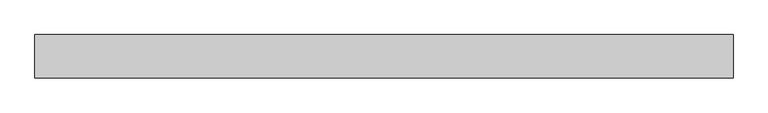
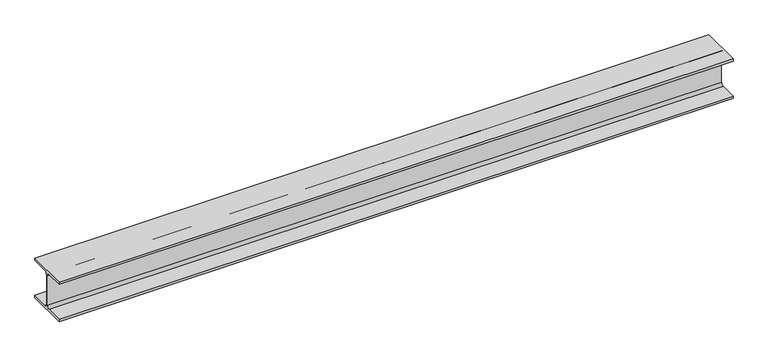
"""IFC4 building model written with IfcOpenShell, lengths in millimetres: beam geometry, 0912_Steel Framing_H-KSD3502 : H_SB_ASB_H-200x200x8x12."""

from ifc_helpers import new_model, si_unit, point, frame, frame_2d, origin, place, context, project, spatial, polyline, circle_curve, trimmed, segment, composite_curve, outline, extrude, source, transform, mapped, element, save


def beam_4c712e8b(model_context):
    return source(origin(), model_context, "Body", "SweptSolid", [
        extrude(outline(composite_curve([segment(polyline([(100.0, -88.0), (100.0, -100.0), (-100.0, -100.0), (-100.0, -88.0), (-17.0, -88.0)]), True, "CONTINUOUS"), segment(trimmed(circle_curve(frame_2d((-17.0, -75.0)), 13.0), [point((-17.0, -88.0))], [point((-4.0, -75.0))], True, "CARTESIAN"), True, "CONTINUOUS"), segment(polyline([(-4.0, -75.0), (-4.0, 75.0)]), True, "CONTINUOUS"), segment(trimmed(circle_curve(frame_2d((-17.0, 75.0)), 13.0), [point((-4.0, 75.0))], [point((-17.0, 88.0))], True, "CARTESIAN"), True, "CONTINUOUS"), segment(polyline([(-17.0, 88.0), (-100.0, 88.0), (-100.0, 100.0), (100.0, 100.0), (100.0, 88.0), (17.0, 88.0)]), True, "CONTINUOUS"), segment(trimmed(circle_curve(frame_2d((17.0, 75.0)), 13.0), [point((17.0, 88.0))], [point((4.0, 75.0))], True, "CARTESIAN"), True, "CONTINUOUS"), segment(polyline([(4.0, 75.0), (4.0, -75.0)]), True, "CONTINUOUS"), segment(trimmed(circle_curve(frame_2d((17.0, -75.0)), 13.0), [point((4.0, -75.0))], [point((17.0, -88.0))], True, "CARTESIAN"), True, "CONTINUOUS"), segment(polyline([(17.0, -88.0), (100.0, -88.0)]), True, "CONTINUOUS")], self_intersect=False)), frame((-1401.7715916, 0.0, 0.0), z_axis=(1.0, 0.0, 0.0), x_axis=(0.0, 1.0, 0.0)), (0.0, 0.0, 1.0), 3222.9601335),
    ])


if __name__ == "__main__":
    model = new_model("IFC4")
    model_context = context("Model", 3, world=origin())
    ifc_project = project(units=[si_unit("LENGTHUNIT", "METRE", prefix="MILLI")], contexts=[model_context])
    site = spatial("IfcSite", under=ifc_project)
    building = spatial("IfcBuilding", under=site)
    placement = place(None, origin())
    beam_shape = beam_4c712e8b(model_context)
    element("IfcBeam", 1, ObjectType="0912_Steel Framing_H-KSD3502 : H_SB_ASB_H-200x200x8x12", at=placement, inside=building, context=model_context, shape_type="MappedRepresentation", body=[
        mapped(beam_shape, transform((0.0, 0.0, 0.0), x_axis=(1.0, 0.0, 0.0), y_axis=(0.0, 1.0, 0.0), z_axis=(0.0, 0.0, 1.0))),
    ])
    save(model, "model.ifc")

# Revit data of these elements
# Type "0912_Steel Framing_H-KSD3502 : H_SB_ASB_H-200x200x8x12"
#   H_WM Code_1 = "S01AA002-00001 | Main Steel Structure Fabrication Work | Shelter/Building | Medium Steel - Standard (90KG/M>Weight≥30KG/M) | Material: (   )"
#   H_WM Code_2 = "S03AA028-00001 | Main Steel Structure Erection Work | Shelter/Building | Medium Steel (90KG/M>Weight≥30KG/M) | Material: (   )"
#   H_WM Code_3 = "S01AA010-00001 | Main Steel Structure Fabrication Work | Shelter/Building | Steel Painting/Coating | for Non-Fireproofed Steel Surface, Surface Preparation, Primer, Second & Final Coat | Material: (   )"
#   H_Q'ty Cal Type Tag = "SB-Q2"
#   Width = 20.0 cm
#   Web Thickness = 0.8 cm
#   Web Fillet = 1.3 cm
#   Warping Constant = 141000.0 cm⁶
#   W = 0
#   Torsional Moment of Inertia = 26.2485 cm⁴
#   Section Area = 63.53 cm²
#   Plastic Modulus weak axis = 244.0 cm³
#   Plastic Modulus strong axis = 525.0 cm³
#   Perimeter = 1.16 m²/m
#   Nominal Weight = 49.90 kgf/m
#   Moment of Inertia weak axis = 1600.00 cm⁴
#   Moment of Inertia strong axis = 4720.00 cm⁴
#   Height = 20.0 cm
#   Flange Thickness = 1.2 cm
#   Elastic Modulus weak axis = 160.0 cm³
#   Elastic Modulus strong axis = 472.0 cm³
#   Centroid Vertical = 10.0 cm
#   Centroid Horizontal = 10.0 cm
#   Ix = 47200000
#   Length [instance default] = 1.5240 m
#   Zx = 525000
#   b = 0.2000 m
#   h = 0.2000 m
#   r = 0.0130 m
#   s = 0.0080 m
#   t = 0.0120 m
#   A = 0.006353 m²
#   Structural Material [instance default] = Steel, 45-345
#   Assembly Code = ""
# Element 1 (IfcBeam, "0912_Steel Framing_H-KSD3502 : H_SB_ASB_H-200x200x8x12")
#   Structural Material = none
# Materials
#   "Steel, 45-345": class "Metal", colour RGB 189 187 185, transparency 0, Description = "Steel 345 MPa", Cost = 0
